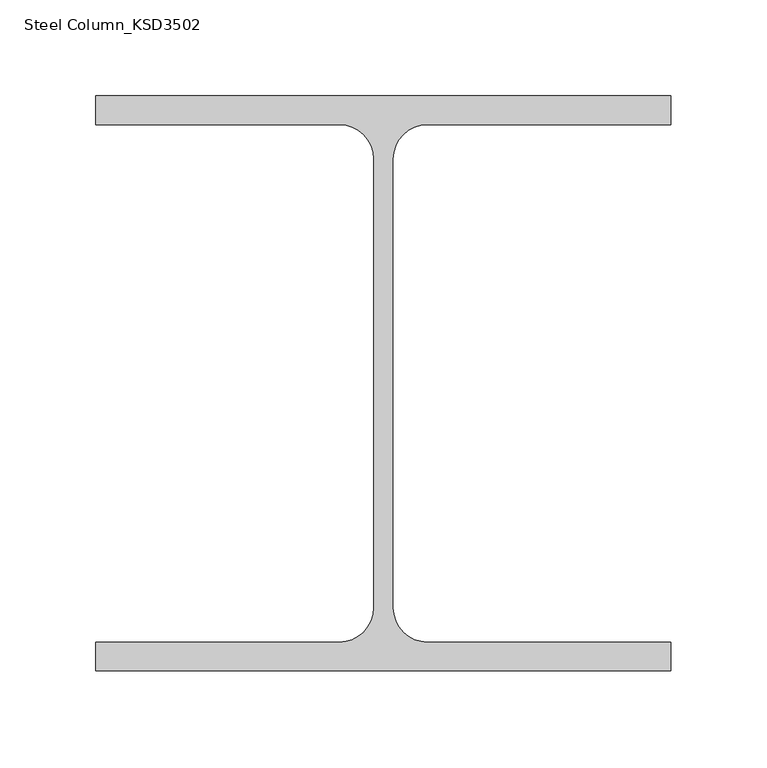
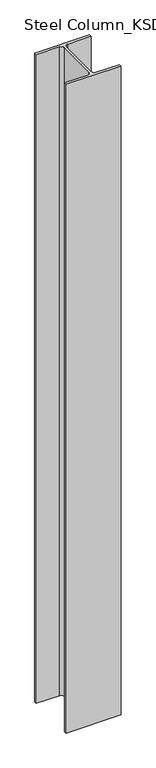
"""IFC4 building model written with IfcOpenShell, lengths in millimetres: column geometry, Steel Column_KSD3502 : H_SC_ASC_H-300×300x10x15."""

import ifcopenshell
import ifcopenshell.guid

model = None  # the IFC model being written
_history = None  # IfcOwnerHistory: only IFC2X3 demands one
_inside = {}  # id of a spatial element -> (the spatial element, [elements in it])
_under = {}  # id of a project, library or spatial element -> (it, [spatial elements below it])
_declared = {}  # id of a project -> (the project, [libraries it declares])
_typed = {}  # id of a type object -> (the type object, [elements of that type])
_made_of = {}  # id of a material, layer set ... -> (it, [elements and type objects made of it])


def new_model(schema):
    """Start an empty IFC model of exactly this schema.

    Asked for "IFC4X3", IfcOpenShell would pick the latest addendum, in which some entities
    have other attributes; the version numbers below select the first issue.
    IFC2X3 requires an IfcOwnerHistory on every rooted entity: one is made here for all.
    """
    global model, _history
    if schema == "IFC4X3":
        model = ifcopenshell.file(schema_version=(4, 3, 0, 0))
    else:
        model = ifcopenshell.file(schema=schema)
    _inside.clear()
    _under.clear()
    _declared.clear()
    _typed.clear()
    _made_of.clear()
    _history = None
    if model.schema == "IFC2X3":
        org = make("IfcOrganization", Name="unknown")
        user = make(
            "IfcPersonAndOrganization",
            ThePerson=make("IfcPerson", FamilyName="unknown"),
            TheOrganization=org,
        )
        app = make(
            "IfcApplication",
            ApplicationDeveloper=org,
            Version="unknown",
            ApplicationFullName="unknown",
            ApplicationIdentifier="unknown",
        )
        _history = make(
            "IfcOwnerHistory",
            OwningUser=user,
            OwningApplication=app,
            ChangeAction="ADDED",
            CreationDate=0,
        )
    return model


def make(cls, **values):
    """One entity of the class cls with the attributes given. An attribute that is None is left unset."""
    return model.create_entity(
        cls, **{name: value for name, value in values.items() if value is not None}
    )


def rooted(cls, **values):
    """An entity with a GlobalId (a new one), such as an element, a storey or a relation."""
    return make(cls, GlobalId=ifcopenshell.guid.new(), OwnerHistory=_history, **values)


def si_unit(unit_type, name, prefix=None):
    """IfcSIUnit, for example si_unit("LENGTHUNIT", "METRE", prefix="MILLI")."""
    return make("IfcSIUnit", UnitType=unit_type, Prefix=prefix, Name=name)


def assignment(units):
    """IfcUnitAssignment: the units of a project."""
    return None if units is None else make("IfcUnitAssignment", Units=units)


def point(xyz):
    """IfcCartesianPoint."""
    return None if xyz is None else make("IfcCartesianPoint", Coordinates=xyz)


def direction(xyz):
    """IfcDirection."""
    return None if xyz is None else make("IfcDirection", DirectionRatios=xyz)


def frame(location, z_axis=None, x_axis=None):
    """IfcAxis2Placement3D, a coordinate frame: its origin and axes. An axis left out is left unset."""
    return make(
        "IfcAxis2Placement3D",
        Location=point(location),
        Axis=direction(z_axis),
        RefDirection=direction(x_axis),
    )


def frame_2d(location, x_axis=None):
    """IfcAxis2Placement2D, a coordinate frame in the plane: its origin and x axis."""
    return make(
        "IfcAxis2Placement2D", Location=point(location), RefDirection=direction(x_axis)
    )


def origin():
    """The frame at (0, 0, 0) with its axes left unset."""
    return frame((0.0, 0.0, 0.0))


def place(relative_to, where):
    """IfcLocalPlacement: puts the frame where relative to a parent placement (None: the world)."""
    return make(
        "IfcLocalPlacement", PlacementRelTo=relative_to, RelativePlacement=where
    )


def context(
    kind, dimensions, precision=None, world=None, true_north=None, identifier=None
):
    """IfcGeometricRepresentationContext, for example the 3D "Model" context."""
    return make(
        "IfcGeometricRepresentationContext",
        ContextIdentifier=identifier,
        ContextType=kind,
        CoordinateSpaceDimension=dimensions,
        Precision=precision,
        WorldCoordinateSystem=world,
        TrueNorth=true_north,
    )


def project(units=None, contexts=None):
    """IfcProject with its units and contexts."""
    return rooted(
        "IfcProject",
        Name="project",
        RepresentationContexts=contexts,
        UnitsInContext=assignment(units),
    )


def spatial(cls, under=None, at=None, **own):
    """A site, building, storey or space (cls), placed at a placement, below another one or the project."""
    s = rooted(cls, ObjectPlacement=at, **own)
    if under is not None:
        _under.setdefault(under.id(), (under, []))[1].append(s)
    return s


def polyline(points):
    """IfcPolyline through the points."""
    return make("IfcPolyline", Points=[point(p) for p in points])


def circle_curve(where, radius):
    """IfcCircle in the frame where."""
    return make("IfcCircle", Position=where, Radius=radius)


def trimmed(basis, trim1, trim2, sense, master):
    """IfcTrimmedCurve: the piece of a basis curve between two trims."""
    return make(
        "IfcTrimmedCurve",
        BasisCurve=basis,
        Trim1=trim1,
        Trim2=trim2,
        SenseAgreement=sense,
        MasterRepresentation=master,
    )


def segment(curve, same_sense, transition):
    """IfcCompositeCurveSegment."""
    return make(
        "IfcCompositeCurveSegment",
        Transition=transition,
        SameSense=same_sense,
        ParentCurve=curve,
    )


def composite_curve(segments, self_intersect=None):
    """IfcCompositeCurve: segments joined end to end."""
    return make("IfcCompositeCurve", Segments=segments, SelfIntersect=self_intersect)


def outline(outer, holes=None, kind="AREA"):
    """IfcArbitraryClosedProfileDef: a profile drawn as a closed curve; with holes, ...WithVoids."""
    if holes is None:
        return make("IfcArbitraryClosedProfileDef", ProfileType=kind, OuterCurve=outer)
    return make(
        "IfcArbitraryProfileDefWithVoids",
        ProfileType=kind,
        OuterCurve=outer,
        InnerCurves=holes,
    )


def extrude(swept, where, along, depth):
    """IfcExtrudedAreaSolid: the profile swept, set in the frame where, extruded along a direction by depth."""
    return make(
        "IfcExtrudedAreaSolid",
        SweptArea=swept,
        Position=where,
        ExtrudedDirection=direction(along),
        Depth=depth,
    )


def shape(context_of_items, identifier, shape_type, items):
    """IfcShapeRepresentation: the items that make up one representation, for example the "Body"."""
    return make(
        "IfcShapeRepresentation",
        ContextOfItems=context_of_items,
        RepresentationIdentifier=identifier,
        RepresentationType=shape_type,
        Items=items,
    )


def source(mapping_origin, context_of_items, identifier, shape_type, items):
    """IfcRepresentationMap: a shape defined once, which mapped items show again and again."""
    return make(
        "IfcRepresentationMap",
        MappingOrigin=mapping_origin,
        MappedRepresentation=shape(context_of_items, identifier, shape_type, items),
    )


def transform(
    local_origin,
    x_axis=None,
    y_axis=None,
    z_axis=None,
    scale=None,
    scale2=None,
    scale3=None,
    uniform=True,
):
    """IfcCartesianTransformationOperator3D, or its non-uniform kind. x_axis, y_axis, z_axis: its Axis1, 2, 3."""
    if uniform:
        return make(
            "IfcCartesianTransformationOperator3D",
            Axis1=direction(x_axis),
            Axis2=direction(y_axis),
            LocalOrigin=point(local_origin),
            Scale=scale,
            Axis3=direction(z_axis),
        )
    return make(
        "IfcCartesianTransformationOperator3DnonUniform",
        Axis1=direction(x_axis),
        Axis2=direction(y_axis),
        LocalOrigin=point(local_origin),
        Scale=scale,
        Axis3=direction(z_axis),
        Scale2=scale2,
        Scale3=scale3,
    )


def mapped(mapping_source, mapping_target):
    """IfcMappedItem: shows the shape of a source again, moved by a transform."""
    return make(
        "IfcMappedItem", MappingSource=mapping_source, MappingTarget=mapping_target
    )


def made_of(thing, what):
    """Note that an element or type object is made of a material, layer set ...; save() writes the relation."""
    if what is not None:
        _made_of.setdefault(what.id(), (what, []))[1].append(thing)
    return thing


def element(
    cls,
    number,
    at=None,
    inside=None,
    cuts=None,
    type_object=None,
    material=None,
    context=None,
    identifier="Body",
    shape_type=None,
    held_by="IfcProductDefinitionShape",
    body=None,
    shapes=None,
    **own,
):
    """One element of the class cls, such as IfcWall. Its Tag is "e" and its number.

    at: its placement. inside: the storey or other place that contains it. cuts: it is an
    opening in that element (IfcRelVoidsElement). A single representation is given by context,
    identifier, shape_type and body (its items); several are given by shapes. held_by: the class
    of the entity that holds the representations. save() writes the other relations.
    """
    e = rooted(cls, Tag="e%d" % number, ObjectPlacement=at, **own)
    if body is not None:
        shapes = [shape(context, identifier, shape_type, body)]
    if shapes is not None:
        e.Representation = make(held_by, Representations=shapes)
    if inside is not None:
        _inside.setdefault(inside.id(), (inside, []))[1].append(e)
    if cuts is not None:
        rooted(
            "IfcRelVoidsElement", RelatingBuildingElement=cuts, RelatedOpeningElement=e
        )
    if type_object is not None:
        _typed.setdefault(type_object.id(), (type_object, []))[1].append(e)
    return made_of(e, material)


def aggregate(whole, parts):
    """IfcRelAggregates: a whole, such as a stair, and the parts it consists of."""
    return rooted("IfcRelAggregates", RelatingObject=whole, RelatedObjects=parts)


def save(model, path):
    """Write the relations noted so far, then the file.

    IfcRelAggregates (storeys below a building ...), IfcRelContainedInSpatialStructure (elements
    in a storey), IfcRelDefinesByType, IfcRelAssociatesMaterial and IfcRelDeclares: one each for
    every whole, place, type object, material and project.
    """
    for whole, parts in _under.values():
        aggregate(whole, parts)
    for where, things in _inside.values():
        rooted(
            "IfcRelContainedInSpatialStructure",
            RelatedElements=things,
            RelatingStructure=where,
        )
    for kind, things in _typed.values():
        rooted("IfcRelDefinesByType", RelatedObjects=things, RelatingType=kind)
    for what, things in _made_of.values():
        rooted("IfcRelAssociatesMaterial", RelatedObjects=things, RelatingMaterial=what)
    for by, libraries in _declared.values():
        rooted("IfcRelDeclares", RelatingContext=by, RelatedDefinitions=libraries)
    model.write(path)


def steel_column_ksd3502_2bf4f364(model_context):
    return source(origin(), model_context, "Body", "SweptSolid", [
        extrude(outline(composite_curve([segment(polyline([(150.0, 150.0), (150.0, 135.0), (23.0, 135.0)]), True, "CONTINUOUS"), segment(trimmed(circle_curve(frame_2d((23.0, 117.0)), 18.0), [point((23.0, 135.0))], [point((5.0, 117.0))], True, "CARTESIAN"), True, "CONTINUOUS"), segment(polyline([(5.0, 117.0), (5.0, -117.0)]), True, "CONTINUOUS"), segment(trimmed(circle_curve(frame_2d((23.0, -117.0)), 18.0), [point((5.0, -117.0))], [point((23.0, -135.0))], True, "CARTESIAN"), True, "CONTINUOUS"), segment(polyline([(23.0, -135.0), (150.0, -135.0), (150.0, -150.0), (-150.0, -150.0), (-150.0, -135.0), (-23.0, -135.0)]), True, "CONTINUOUS"), segment(trimmed(circle_curve(frame_2d((-23.0, -117.0)), 18.0), [point((-23.0, -135.0))], [point((-5.0, -117.0))], True, "CARTESIAN"), True, "CONTINUOUS"), segment(polyline([(-5.0, -117.0), (-5.0, 117.0)]), True, "CONTINUOUS"), segment(trimmed(circle_curve(frame_2d((-23.0, 117.0)), 18.0), [point((-5.0, 117.0))], [point((-23.0, 135.0))], True, "CARTESIAN"), True, "CONTINUOUS"), segment(polyline([(-23.0, 135.0), (-150.0, 135.0), (-150.0, 150.0), (150.0, 150.0)]), True, "CONTINUOUS")], self_intersect=False)), frame((0.0, 0.0, 685.9720055), z_axis=(0.0, 0.0, 1.0), x_axis=(1.0, 0.0, 0.0)), (0.0, 0.0, 1.0), 3764.0),
    ])


if __name__ == "__main__":
    model = new_model("IFC4")
    model_context = context("Model", 3, world=origin())
    ifc_project = project(units=[si_unit("LENGTHUNIT", "METRE", prefix="MILLI")], contexts=[model_context])
    site = spatial("IfcSite", under=ifc_project)
    building = spatial("IfcBuilding", under=site)
    placement = place(None, origin())
    steel_column_ksd3502_shape = steel_column_ksd3502_2bf4f364(model_context)
    element("IfcColumn", 1, ObjectType="Steel Column_KSD3502 : H_SC_ASC_H-300×300x10x15", at=placement, inside=building, context=model_context, shape_type="MappedRepresentation", body=[
        mapped(steel_column_ksd3502_shape, transform((0.0, 0.0, 0.0), x_axis=(1.0, 0.0, 0.0), y_axis=(0.0, 1.0, 0.0), z_axis=(0.0, 0.0, 1.0))),
    ])
    save(model, "model.ifc")

# Revit data of these elements
# Type "Steel Column_KSD3502 : H_SC_ASC_H-300×300x10x15"
#   Width = 30.0 cm
#   Web Thickness = 1.0 cm
#   Web Fillet = 1.8 cm
#   Warping Constant = 1370670.0 cm⁶
#   Torsional Moment of Inertia = 77.00 cm⁴
#   Section Area = 119.8 cm²
#   Plastic Modulus weak axis = 684.0 cm³
#   Plastic Modulus strong axis = 1500.0 cm³
#   Perimeter = 1.27 m²/m
#   Nominal Weight = 94.00 kgf/m
#   Moment of Inertia weak axis = 6750.00 cm⁴
#   Moment of Inertia strong axis = 20400.00 cm⁴
#   Height = 30.0 cm
#   Flange Thickness = 1.5 cm
#   Elastic Modulus weak axis = 450.0 cm³
#   Elastic Modulus strong axis = 1360.0 cm³
#   Centroid Vertical = 15.0 cm
#   Centroid Horizontal = 15.0 cm
#   Bolt Spacing = 13.97 cm
#   Structural Material [instance default] = Steel, 45-345
#   Section Name Key = ""
#   Assembly Code = ""
# Element 1 (IfcColumn, "Steel Column_KSD3502 : H_SC_ASC_H-300×300x10x15")
#   Structural Material = none
# Materials
#   "Steel, 45-345": class "Metal", colour RGB 189 187 185, transparency 0, Description = "Steel 345 MPa", Cost = 0
